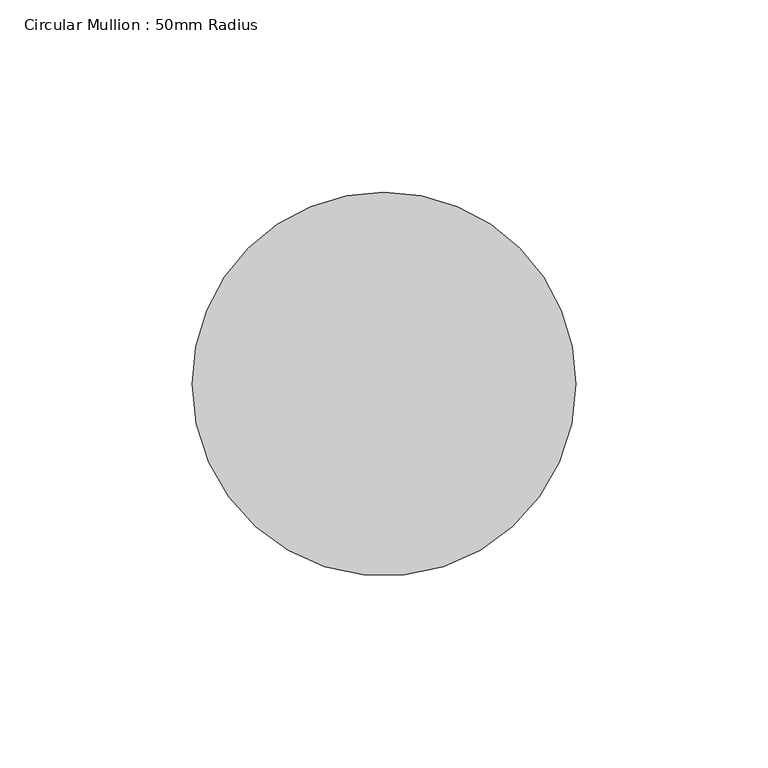
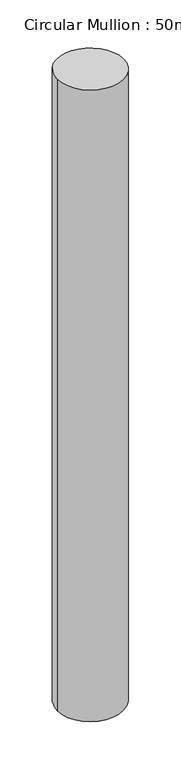
"""IFC4 building model written with IfcOpenShell, lengths in millimetres: member geometry, Circular Mullion : 50mm Radius."""

from ifc_helpers import new_model, si_unit, frame, origin, place, context, project, spatial, ellipse_curve, source, transform, mapped, element, save
from ifc_brep_helpers import plane_surface, cylinder_surface, advanced_brep


def circular_mullion_50mm_radius_9c7080d7(model_context):
    return source(origin(), model_context, "Body", "AdvancedBrep", [
        advanced_brep(
        [(-100.0, 0.0, 2.2092613), (0.0, 0.0, 0.0), (0.0, 0.0, -1004.3847291), (-100.0, 0.0, -1006.6203123)],
        [
            (0, 1, ellipse_curve(frame((-50.0, 0.0, 1.1046306), z_axis=(-0.02208174400178452, -0.02227318434112407, -0.999508029903285), x_axis=(-0.7037019086496239, -0.7098027371066011, 0.031363962741556964)), 50.0246106, 50.0)),
            (1, 2),
            (2, 3, ellipse_curve(frame((-50.0, 0.0, -1005.5025207), z_axis=(-0.022344569542256488, -0.022538288479276, 0.9994962459981509), x_axis=(0.7036936122114924, 0.7097943687414955, 0.03173726887436507)), 50.0252004, 50.0)),
            (3, 0),
            (1, 0, ellipse_curve(frame((-50.0, 0.0, 1.1046306), z_axis=(-0.02208174400178452, -0.02227318434112407, -0.999508029903285), x_axis=(-0.7037019086496239, -0.7098027371066011, 0.031363962741556964)), 50.0246106, 50.0)),
            (3, 2, ellipse_curve(frame((-50.0, 0.0, -1005.5025207), z_axis=(-0.022344569542256488, -0.022538288479276, 0.9994962459981509), x_axis=(0.7036936122114924, 0.7097943687414955, 0.03173726887436507)), 50.0252004, 50.0)),
        ],
        [
            cylinder_surface(frame((-50.0, 0.0, 0.0), z_axis=(0.0, 0.0, 1.0), x_axis=(1.0, 0.0, 0.0)), 50.0),
            plane_surface(frame((-216.4543633, 214.5939155, 0.0), z_axis=(0.02208174400178452, 0.02227318434112407, 0.999508029903285), x_axis=(0.7037019086496235, 0.7098027371066014, -0.03136396274156123))),
            plane_surface(frame((-216.4543633, 214.5939155, -1004.3847291), z_axis=(0.022344569542256488, 0.022538288479276, -0.9994962459981509), x_axis=(0.7036936122114923, 0.7097943687414955, 0.03173726887436601))),
        ],
        [
            (0, [[1, 2, 3, 4]]),
            (0, [[5, -4, 6, -2]]),
            (1, [[-1, -5]]),
            (2, [[-6, -3]]),
        ],
    ),
    ])


if __name__ == "__main__":
    model = new_model("IFC4")
    model_context = context("Model", 3, world=origin())
    ifc_project = project(units=[si_unit("LENGTHUNIT", "METRE", prefix="MILLI")], contexts=[model_context])
    site = spatial("IfcSite", under=ifc_project)
    building = spatial("IfcBuilding", under=site)
    placement = place(None, origin())
    circular_mullion_50mm_radius_shape = circular_mullion_50mm_radius_9c7080d7(model_context)
    element("IfcMember", 1, ObjectType="Circular Mullion : 50mm Radius", at=placement, inside=building, context=model_context, shape_type="MappedRepresentation", body=[
        mapped(circular_mullion_50mm_radius_shape, transform((0.0, 0.0, 0.0), x_axis=(1.0, 0.0, 0.0), y_axis=(0.0, 1.0, 0.0), z_axis=(0.0, 0.0, 1.0))),
    ])
    save(model, "model.ifc")

# Revit data of these elements
# Type "Circular Mullion : 50mm Radius"
#   built-in parameter 1007350 = 0.164042 (stored number, unit not read)
# Element 1 (IfcMember, "Circular Mullion : 50mm Radius")
#   Materials on its faces: "Aluminium"
# Materials
#   "Aluminium": class "Metal", colour RGB 247 247 247, transparency 0, Description = "Aluminium 6061", Cost = 0
